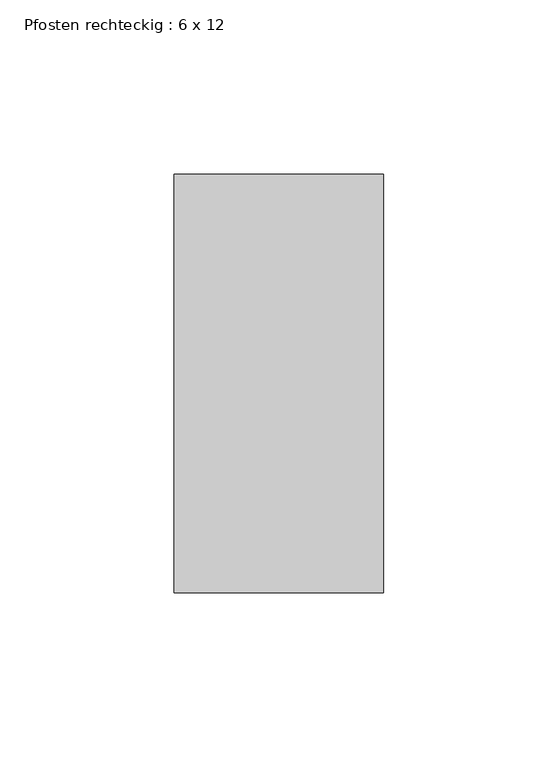
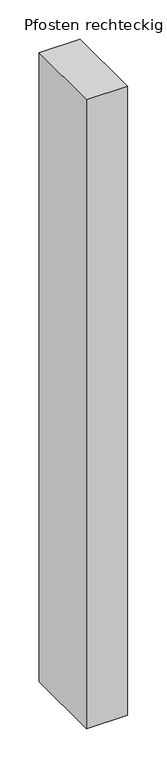
"""IFC4 building model written with IfcOpenShell, lengths in millimetres: member geometry, Pfosten rechteckig : 6 x 12."""

from ifc_helpers import new_model, si_unit, frame, origin, place, context, project, spatial, polyline, outline, extrude, source, transform, mapped, element, save


def pfosten_rechteckig_6_x_12_940153c9(model_context):
    return source(origin(), model_context, "Body", "SweptSolid", [
        extrude(outline(polyline([(0.0, 60.0), (0.0, -60.0), (-60.0, -60.0), (-60.0, 60.0), (0.0, 60.0)])), frame((0.0, 0.0, -973.2237978), z_axis=(0.0, 0.0, 1.0), x_axis=(1.0, 0.0, 0.0)), (0.0, 0.0, 1.0), 973.2237978),
    ])


if __name__ == "__main__":
    model = new_model("IFC4")
    model_context = context("Model", 3, world=origin())
    ifc_project = project(units=[si_unit("LENGTHUNIT", "METRE", prefix="MILLI")], contexts=[model_context])
    site = spatial("IfcSite", under=ifc_project)
    building = spatial("IfcBuilding", under=site)
    placement = place(None, origin())
    pfosten_rechteckig_6_x_12_shape = pfosten_rechteckig_6_x_12_940153c9(model_context)
    element("IfcMember", 1, ObjectType="Pfosten rechteckig : 6 x 12", at=placement, inside=building, context=model_context, shape_type="MappedRepresentation", body=[
        mapped(pfosten_rechteckig_6_x_12_shape, transform((0.0, 0.0, 0.0), x_axis=(1.0, 0.0, 0.0), y_axis=(0.0, 1.0, 0.0), z_axis=(0.0, 0.0, 1.0))),
    ])
    save(model, "model.ifc")

# Revit data of these elements
# Type "Pfosten rechteckig : 6 x 12"
#   built-in parameter 1007304 = 0.393701 (stored number, unit not read)
#   built-in parameter 1007301 = 0.0984252 (stored number, unit not read)
#   built-in parameter 1007300 = 0.0984252 (stored number, unit not read)
# Element 1 (IfcMember, "Pfosten rechteckig : 6 x 12")
#   Materials on its faces: "Metall - verzinkt"
# Materials
#   "Metall - verzinkt": class "Allgemeines", colour RGB 200 200 200, transparency 0, Cost = 0
